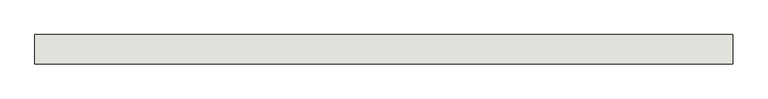
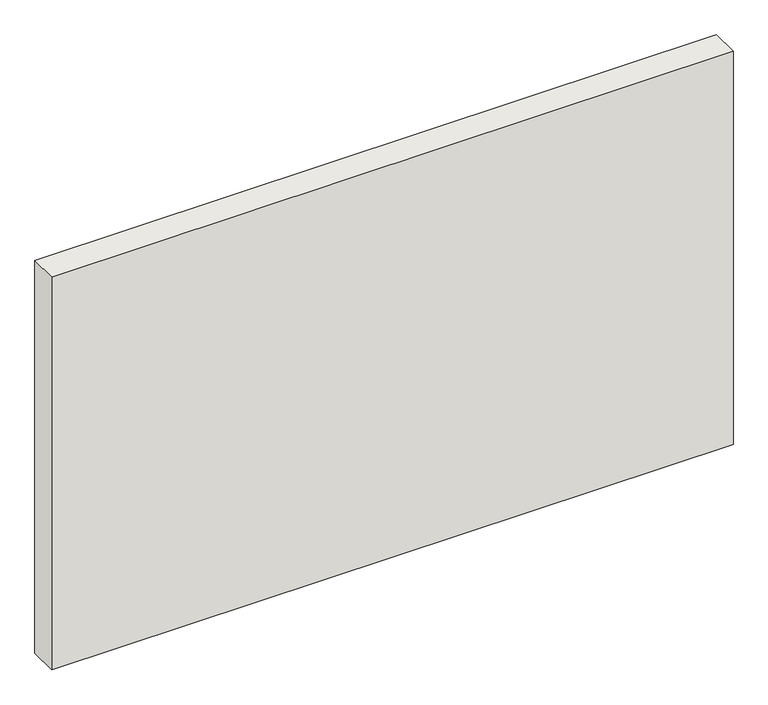
"""IFC4 building model written with IfcOpenShell, lengths in millimetres: wall geometry, Holzwand."""

import ifcopenshell
import ifcopenshell.guid

model = None  # the IFC model being written
_history = None  # IfcOwnerHistory: only IFC2X3 demands one
_inside = {}  # id of a spatial element -> (the spatial element, [elements in it])
_under = {}  # id of a project, library or spatial element -> (it, [spatial elements below it])
_declared = {}  # id of a project -> (the project, [libraries it declares])
_typed = {}  # id of a type object -> (the type object, [elements of that type])
_made_of = {}  # id of a material, layer set ... -> (it, [elements and type objects made of it])


def new_model(schema):
    """Start an empty IFC model of exactly this schema.

    Asked for "IFC4X3", IfcOpenShell would pick the latest addendum, in which some entities
    have other attributes; the version numbers below select the first issue.
    IFC2X3 requires an IfcOwnerHistory on every rooted entity: one is made here for all.
    """
    global model, _history
    if schema == "IFC4X3":
        model = ifcopenshell.file(schema_version=(4, 3, 0, 0))
    else:
        model = ifcopenshell.file(schema=schema)
    _inside.clear()
    _under.clear()
    _declared.clear()
    _typed.clear()
    _made_of.clear()
    _history = None
    if model.schema == "IFC2X3":
        org = make("IfcOrganization", Name="unknown")
        user = make(
            "IfcPersonAndOrganization",
            ThePerson=make("IfcPerson", FamilyName="unknown"),
            TheOrganization=org,
        )
        app = make(
            "IfcApplication",
            ApplicationDeveloper=org,
            Version="unknown",
            ApplicationFullName="unknown",
            ApplicationIdentifier="unknown",
        )
        _history = make(
            "IfcOwnerHistory",
            OwningUser=user,
            OwningApplication=app,
            ChangeAction="ADDED",
            CreationDate=0,
        )
    return model


def make(cls, **values):
    """One entity of the class cls with the attributes given. An attribute that is None is left unset."""
    return model.create_entity(
        cls, **{name: value for name, value in values.items() if value is not None}
    )


def rooted(cls, **values):
    """An entity with a GlobalId (a new one), such as an element, a storey or a relation."""
    return make(cls, GlobalId=ifcopenshell.guid.new(), OwnerHistory=_history, **values)


def si_unit(unit_type, name, prefix=None):
    """IfcSIUnit, for example si_unit("LENGTHUNIT", "METRE", prefix="MILLI")."""
    return make("IfcSIUnit", UnitType=unit_type, Prefix=prefix, Name=name)


def assignment(units):
    """IfcUnitAssignment: the units of a project."""
    return None if units is None else make("IfcUnitAssignment", Units=units)


def point(xyz):
    """IfcCartesianPoint."""
    return None if xyz is None else make("IfcCartesianPoint", Coordinates=xyz)


def direction(xyz):
    """IfcDirection."""
    return None if xyz is None else make("IfcDirection", DirectionRatios=xyz)


def frame(location, z_axis=None, x_axis=None):
    """IfcAxis2Placement3D, a coordinate frame: its origin and axes. An axis left out is left unset."""
    return make(
        "IfcAxis2Placement3D",
        Location=point(location),
        Axis=direction(z_axis),
        RefDirection=direction(x_axis),
    )


def origin():
    """The frame at (0, 0, 0) with its axes left unset."""
    return frame((0.0, 0.0, 0.0))


def origin_with_axes():
    """The frame at (0, 0, 0) with the z axis (0, 0, 1) and the x axis (1, 0, 0) written out."""
    return frame((0.0, 0.0, 0.0), z_axis=(0.0, 0.0, 1.0), x_axis=(1.0, 0.0, 0.0))


def place(relative_to, where):
    """IfcLocalPlacement: puts the frame where relative to a parent placement (None: the world)."""
    return make(
        "IfcLocalPlacement", PlacementRelTo=relative_to, RelativePlacement=where
    )


def context(
    kind, dimensions, precision=None, world=None, true_north=None, identifier=None
):
    """IfcGeometricRepresentationContext, for example the 3D "Model" context."""
    return make(
        "IfcGeometricRepresentationContext",
        ContextIdentifier=identifier,
        ContextType=kind,
        CoordinateSpaceDimension=dimensions,
        Precision=precision,
        WorldCoordinateSystem=world,
        TrueNorth=true_north,
    )


def project(units=None, contexts=None):
    """IfcProject with its units and contexts."""
    return rooted(
        "IfcProject",
        Name="project",
        RepresentationContexts=contexts,
        UnitsInContext=assignment(units),
    )


def spatial(cls, under=None, at=None, **own):
    """A site, building, storey or space (cls), placed at a placement, below another one or the project."""
    s = rooted(cls, ObjectPlacement=at, **own)
    if under is not None:
        _under.setdefault(under.id(), (under, []))[1].append(s)
    return s


def polyline(points):
    """IfcPolyline through the points."""
    return make("IfcPolyline", Points=[point(p) for p in points])


def outline(outer, holes=None, kind="AREA"):
    """IfcArbitraryClosedProfileDef: a profile drawn as a closed curve; with holes, ...WithVoids."""
    if holes is None:
        return make("IfcArbitraryClosedProfileDef", ProfileType=kind, OuterCurve=outer)
    return make(
        "IfcArbitraryProfileDefWithVoids",
        ProfileType=kind,
        OuterCurve=outer,
        InnerCurves=holes,
    )


def extrude(swept, where, along, depth):
    """IfcExtrudedAreaSolid: the profile swept, set in the frame where, extruded along a direction by depth."""
    return make(
        "IfcExtrudedAreaSolid",
        SweptArea=swept,
        Position=where,
        ExtrudedDirection=direction(along),
        Depth=depth,
    )


def shape(context_of_items, identifier, shape_type, items):
    """IfcShapeRepresentation: the items that make up one representation, for example the "Body"."""
    return make(
        "IfcShapeRepresentation",
        ContextOfItems=context_of_items,
        RepresentationIdentifier=identifier,
        RepresentationType=shape_type,
        Items=items,
    )


def source(mapping_origin, context_of_items, identifier, shape_type, items):
    """IfcRepresentationMap: a shape defined once, which mapped items show again and again."""
    return make(
        "IfcRepresentationMap",
        MappingOrigin=mapping_origin,
        MappedRepresentation=shape(context_of_items, identifier, shape_type, items),
    )


def transform(
    local_origin,
    x_axis=None,
    y_axis=None,
    z_axis=None,
    scale=None,
    scale2=None,
    scale3=None,
    uniform=True,
):
    """IfcCartesianTransformationOperator3D, or its non-uniform kind. x_axis, y_axis, z_axis: its Axis1, 2, 3."""
    if uniform:
        return make(
            "IfcCartesianTransformationOperator3D",
            Axis1=direction(x_axis),
            Axis2=direction(y_axis),
            LocalOrigin=point(local_origin),
            Scale=scale,
            Axis3=direction(z_axis),
        )
    return make(
        "IfcCartesianTransformationOperator3DnonUniform",
        Axis1=direction(x_axis),
        Axis2=direction(y_axis),
        LocalOrigin=point(local_origin),
        Scale=scale,
        Axis3=direction(z_axis),
        Scale2=scale2,
        Scale3=scale3,
    )


def mapped(mapping_source, mapping_target):
    """IfcMappedItem: shows the shape of a source again, moved by a transform."""
    return make(
        "IfcMappedItem", MappingSource=mapping_source, MappingTarget=mapping_target
    )


def made_of(thing, what):
    """Note that an element or type object is made of a material, layer set ...; save() writes the relation."""
    if what is not None:
        _made_of.setdefault(what.id(), (what, []))[1].append(thing)
    return thing


def element(
    cls,
    number,
    at=None,
    inside=None,
    cuts=None,
    type_object=None,
    material=None,
    context=None,
    identifier="Body",
    shape_type=None,
    held_by="IfcProductDefinitionShape",
    body=None,
    shapes=None,
    **own,
):
    """One element of the class cls, such as IfcWall. Its Tag is "e" and its number.

    at: its placement. inside: the storey or other place that contains it. cuts: it is an
    opening in that element (IfcRelVoidsElement). A single representation is given by context,
    identifier, shape_type and body (its items); several are given by shapes. held_by: the class
    of the entity that holds the representations. save() writes the other relations.
    """
    e = rooted(cls, Tag="e%d" % number, ObjectPlacement=at, **own)
    if body is not None:
        shapes = [shape(context, identifier, shape_type, body)]
    if shapes is not None:
        e.Representation = make(held_by, Representations=shapes)
    if inside is not None:
        _inside.setdefault(inside.id(), (inside, []))[1].append(e)
    if cuts is not None:
        rooted(
            "IfcRelVoidsElement", RelatingBuildingElement=cuts, RelatedOpeningElement=e
        )
    if type_object is not None:
        _typed.setdefault(type_object.id(), (type_object, []))[1].append(e)
    return made_of(e, material)


def aggregate(whole, parts):
    """IfcRelAggregates: a whole, such as a stair, and the parts it consists of."""
    return rooted("IfcRelAggregates", RelatingObject=whole, RelatedObjects=parts)


def save(model, path):
    """Write the relations noted so far, then the file.

    IfcRelAggregates (storeys below a building ...), IfcRelContainedInSpatialStructure (elements
    in a storey), IfcRelDefinesByType, IfcRelAssociatesMaterial and IfcRelDeclares: one each for
    every whole, place, type object, material and project.
    """
    for whole, parts in _under.values():
        aggregate(whole, parts)
    for where, things in _inside.values():
        rooted(
            "IfcRelContainedInSpatialStructure",
            RelatedElements=things,
            RelatingStructure=where,
        )
    for kind, things in _typed.values():
        rooted("IfcRelDefinesByType", RelatedObjects=things, RelatingType=kind)
    for what, things in _made_of.values():
        rooted("IfcRelAssociatesMaterial", RelatedObjects=things, RelatingMaterial=what)
    for by, libraries in _declared.values():
        rooted("IfcRelDeclares", RelatingContext=by, RelatedDefinitions=libraries)
    model.write(path)


def wall_3bc29835(model_context):
    return source(origin(), model_context, "Body", "SweptSolid", [
        extrude(outline(polyline([(0.0, 200.0), (4720.0, 200.0), (4720.0, 0.0), (0.0, 0.0), (0.0, 200.0)])), origin_with_axes(), (0.0, 0.0, 1.0), 2880.0),
    ])


if __name__ == "__main__":
    model = new_model("IFC4")
    model_context = context("Model", 3, world=origin())
    ifc_project = project(units=[si_unit("LENGTHUNIT", "METRE", prefix="MILLI")], contexts=[model_context])
    site = spatial("IfcSite", under=ifc_project)
    building = spatial("IfcBuilding", under=site)
    placement = place(None, origin())
    wall_shape = wall_3bc29835(model_context)
    element("IfcWall", 1, ObjectType="Holzwand", at=placement, inside=building, context=model_context, shape_type="MappedRepresentation", body=[
        mapped(wall_shape, transform((0.0, 0.0, 0.0), x_axis=(1.0, 0.0, 0.0), y_axis=(0.0, 1.0, 0.0), z_axis=(0.0, 0.0, 1.0))),
    ])
    save(model, "model.ifc")

# Revit data of these elements
# Element 1 (IfcWall, "Holzwand")
#   Materials on its faces: "holzschalung"
# Materials
#   "holzschalung": class "Unassigned", colour RGB 128 128 128, transparency 0
